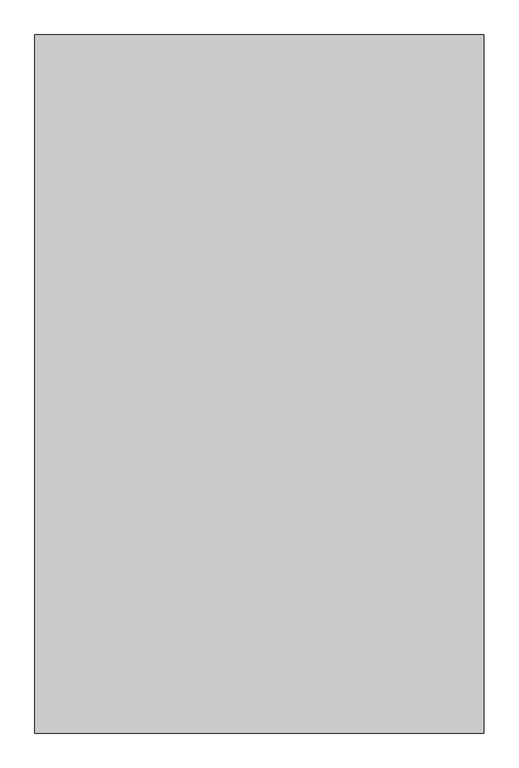
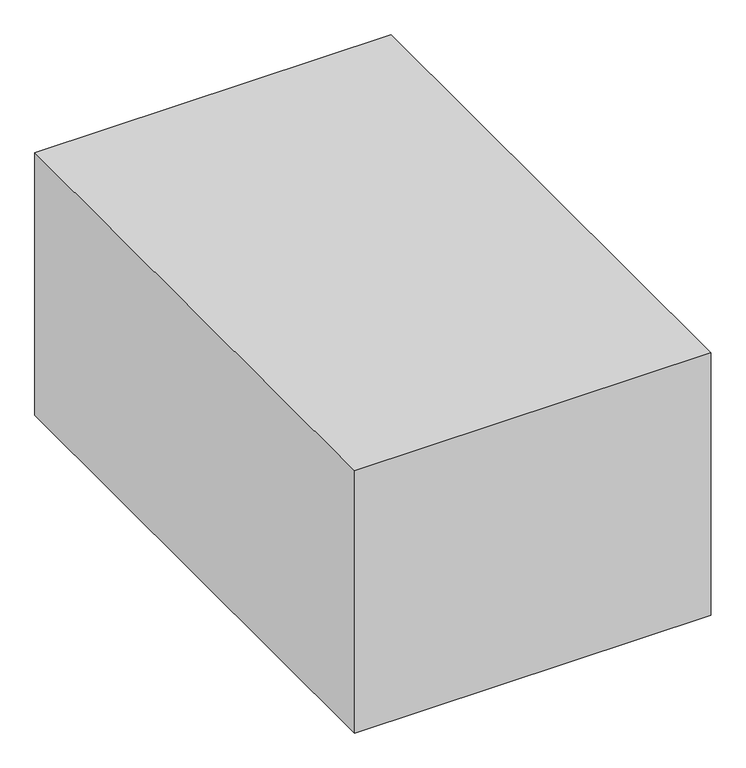
"""IFC4 building model written with IfcOpenShell, lengths in millimetres: proxy geometry, Space Planning Box_hec : Space Planning Box_hec."""

import ifcopenshell
import ifcopenshell.guid

model = None  # the IFC model being written
_history = None  # IfcOwnerHistory: only IFC2X3 demands one
_inside = {}  # id of a spatial element -> (the spatial element, [elements in it])
_under = {}  # id of a project, library or spatial element -> (it, [spatial elements below it])
_declared = {}  # id of a project -> (the project, [libraries it declares])
_typed = {}  # id of a type object -> (the type object, [elements of that type])
_made_of = {}  # id of a material, layer set ... -> (it, [elements and type objects made of it])


def new_model(schema):
    """Start an empty IFC model of exactly this schema.

    Asked for "IFC4X3", IfcOpenShell would pick the latest addendum, in which some entities
    have other attributes; the version numbers below select the first issue.
    IFC2X3 requires an IfcOwnerHistory on every rooted entity: one is made here for all.
    """
    global model, _history
    if schema == "IFC4X3":
        model = ifcopenshell.file(schema_version=(4, 3, 0, 0))
    else:
        model = ifcopenshell.file(schema=schema)
    _inside.clear()
    _under.clear()
    _declared.clear()
    _typed.clear()
    _made_of.clear()
    _history = None
    if model.schema == "IFC2X3":
        org = make("IfcOrganization", Name="unknown")
        user = make(
            "IfcPersonAndOrganization",
            ThePerson=make("IfcPerson", FamilyName="unknown"),
            TheOrganization=org,
        )
        app = make(
            "IfcApplication",
            ApplicationDeveloper=org,
            Version="unknown",
            ApplicationFullName="unknown",
            ApplicationIdentifier="unknown",
        )
        _history = make(
            "IfcOwnerHistory",
            OwningUser=user,
            OwningApplication=app,
            ChangeAction="ADDED",
            CreationDate=0,
        )
    return model


def make(cls, **values):
    """One entity of the class cls with the attributes given. An attribute that is None is left unset."""
    return model.create_entity(
        cls, **{name: value for name, value in values.items() if value is not None}
    )


def rooted(cls, **values):
    """An entity with a GlobalId (a new one), such as an element, a storey or a relation."""
    return make(cls, GlobalId=ifcopenshell.guid.new(), OwnerHistory=_history, **values)


def si_unit(unit_type, name, prefix=None):
    """IfcSIUnit, for example si_unit("LENGTHUNIT", "METRE", prefix="MILLI")."""
    return make("IfcSIUnit", UnitType=unit_type, Prefix=prefix, Name=name)


def assignment(units):
    """IfcUnitAssignment: the units of a project."""
    return None if units is None else make("IfcUnitAssignment", Units=units)


def point(xyz):
    """IfcCartesianPoint."""
    return None if xyz is None else make("IfcCartesianPoint", Coordinates=xyz)


def direction(xyz):
    """IfcDirection."""
    return None if xyz is None else make("IfcDirection", DirectionRatios=xyz)


def frame(location, z_axis=None, x_axis=None):
    """IfcAxis2Placement3D, a coordinate frame: its origin and axes. An axis left out is left unset."""
    return make(
        "IfcAxis2Placement3D",
        Location=point(location),
        Axis=direction(z_axis),
        RefDirection=direction(x_axis),
    )


def origin():
    """The frame at (0, 0, 0) with its axes left unset."""
    return frame((0.0, 0.0, 0.0))


def origin_with_axes():
    """The frame at (0, 0, 0) with the z axis (0, 0, 1) and the x axis (1, 0, 0) written out."""
    return frame((0.0, 0.0, 0.0), z_axis=(0.0, 0.0, 1.0), x_axis=(1.0, 0.0, 0.0))


def place(relative_to, where):
    """IfcLocalPlacement: puts the frame where relative to a parent placement (None: the world)."""
    return make(
        "IfcLocalPlacement", PlacementRelTo=relative_to, RelativePlacement=where
    )


def context(
    kind, dimensions, precision=None, world=None, true_north=None, identifier=None
):
    """IfcGeometricRepresentationContext, for example the 3D "Model" context."""
    return make(
        "IfcGeometricRepresentationContext",
        ContextIdentifier=identifier,
        ContextType=kind,
        CoordinateSpaceDimension=dimensions,
        Precision=precision,
        WorldCoordinateSystem=world,
        TrueNorth=true_north,
    )


def project(units=None, contexts=None):
    """IfcProject with its units and contexts."""
    return rooted(
        "IfcProject",
        Name="project",
        RepresentationContexts=contexts,
        UnitsInContext=assignment(units),
    )


def spatial(cls, under=None, at=None, **own):
    """A site, building, storey or space (cls), placed at a placement, below another one or the project."""
    s = rooted(cls, ObjectPlacement=at, **own)
    if under is not None:
        _under.setdefault(under.id(), (under, []))[1].append(s)
    return s


def polyline(points):
    """IfcPolyline through the points."""
    return make("IfcPolyline", Points=[point(p) for p in points])


def outline(outer, holes=None, kind="AREA"):
    """IfcArbitraryClosedProfileDef: a profile drawn as a closed curve; with holes, ...WithVoids."""
    if holes is None:
        return make("IfcArbitraryClosedProfileDef", ProfileType=kind, OuterCurve=outer)
    return make(
        "IfcArbitraryProfileDefWithVoids",
        ProfileType=kind,
        OuterCurve=outer,
        InnerCurves=holes,
    )


def extrude(swept, where, along, depth):
    """IfcExtrudedAreaSolid: the profile swept, set in the frame where, extruded along a direction by depth."""
    return make(
        "IfcExtrudedAreaSolid",
        SweptArea=swept,
        Position=where,
        ExtrudedDirection=direction(along),
        Depth=depth,
    )


def shape(context_of_items, identifier, shape_type, items):
    """IfcShapeRepresentation: the items that make up one representation, for example the "Body"."""
    return make(
        "IfcShapeRepresentation",
        ContextOfItems=context_of_items,
        RepresentationIdentifier=identifier,
        RepresentationType=shape_type,
        Items=items,
    )


def source(mapping_origin, context_of_items, identifier, shape_type, items):
    """IfcRepresentationMap: a shape defined once, which mapped items show again and again."""
    return make(
        "IfcRepresentationMap",
        MappingOrigin=mapping_origin,
        MappedRepresentation=shape(context_of_items, identifier, shape_type, items),
    )


def transform(
    local_origin,
    x_axis=None,
    y_axis=None,
    z_axis=None,
    scale=None,
    scale2=None,
    scale3=None,
    uniform=True,
):
    """IfcCartesianTransformationOperator3D, or its non-uniform kind. x_axis, y_axis, z_axis: its Axis1, 2, 3."""
    if uniform:
        return make(
            "IfcCartesianTransformationOperator3D",
            Axis1=direction(x_axis),
            Axis2=direction(y_axis),
            LocalOrigin=point(local_origin),
            Scale=scale,
            Axis3=direction(z_axis),
        )
    return make(
        "IfcCartesianTransformationOperator3DnonUniform",
        Axis1=direction(x_axis),
        Axis2=direction(y_axis),
        LocalOrigin=point(local_origin),
        Scale=scale,
        Axis3=direction(z_axis),
        Scale2=scale2,
        Scale3=scale3,
    )


def mapped(mapping_source, mapping_target):
    """IfcMappedItem: shows the shape of a source again, moved by a transform."""
    return make(
        "IfcMappedItem", MappingSource=mapping_source, MappingTarget=mapping_target
    )


def made_of(thing, what):
    """Note that an element or type object is made of a material, layer set ...; save() writes the relation."""
    if what is not None:
        _made_of.setdefault(what.id(), (what, []))[1].append(thing)
    return thing


def element(
    cls,
    number,
    at=None,
    inside=None,
    cuts=None,
    type_object=None,
    material=None,
    context=None,
    identifier="Body",
    shape_type=None,
    held_by="IfcProductDefinitionShape",
    body=None,
    shapes=None,
    **own,
):
    """One element of the class cls, such as IfcWall. Its Tag is "e" and its number.

    at: its placement. inside: the storey or other place that contains it. cuts: it is an
    opening in that element (IfcRelVoidsElement). A single representation is given by context,
    identifier, shape_type and body (its items); several are given by shapes. held_by: the class
    of the entity that holds the representations. save() writes the other relations.
    """
    e = rooted(cls, Tag="e%d" % number, ObjectPlacement=at, **own)
    if body is not None:
        shapes = [shape(context, identifier, shape_type, body)]
    if shapes is not None:
        e.Representation = make(held_by, Representations=shapes)
    if inside is not None:
        _inside.setdefault(inside.id(), (inside, []))[1].append(e)
    if cuts is not None:
        rooted(
            "IfcRelVoidsElement", RelatingBuildingElement=cuts, RelatedOpeningElement=e
        )
    if type_object is not None:
        _typed.setdefault(type_object.id(), (type_object, []))[1].append(e)
    return made_of(e, material)


def aggregate(whole, parts):
    """IfcRelAggregates: a whole, such as a stair, and the parts it consists of."""
    return rooted("IfcRelAggregates", RelatingObject=whole, RelatedObjects=parts)


def save(model, path):
    """Write the relations noted so far, then the file.

    IfcRelAggregates (storeys below a building ...), IfcRelContainedInSpatialStructure (elements
    in a storey), IfcRelDefinesByType, IfcRelAssociatesMaterial and IfcRelDeclares: one each for
    every whole, place, type object, material and project.
    """
    for whole, parts in _under.values():
        aggregate(whole, parts)
    for where, things in _inside.values():
        rooted(
            "IfcRelContainedInSpatialStructure",
            RelatedElements=things,
            RelatingStructure=where,
        )
    for kind, things in _typed.values():
        rooted("IfcRelDefinesByType", RelatedObjects=things, RelatingType=kind)
    for what, things in _made_of.values():
        rooted("IfcRelAssociatesMaterial", RelatedObjects=things, RelatingMaterial=what)
    for by, libraries in _declared.values():
        rooted("IfcRelDeclares", RelatingContext=by, RelatedDefinitions=libraries)
    model.write(path)


def generic_models_10b6925f(model_context):
    return source(origin(), model_context, "Body", "SweptSolid", [
        extrude(outline(polyline([(2250.0, 3500.0), (2250.0, -3500.0), (-2250.0, -3500.0), (-2250.0, 3500.0), (2250.0, 3500.0)])), origin_with_axes(), (0.0, 0.0, 1.0), 3500.0),
    ])


if __name__ == "__main__":
    model = new_model("IFC4")
    model_context = context("Model", 3, world=origin())
    ifc_project = project(units=[si_unit("LENGTHUNIT", "METRE", prefix="MILLI")], contexts=[model_context])
    site = spatial("IfcSite", under=ifc_project)
    building = spatial("IfcBuilding", under=site)
    placement = place(None, origin())
    generic_models_shape = generic_models_10b6925f(model_context)
    element("IfcBuildingElementProxy", 1, Name="Space Planning Box_hec : Space Planning Box_hec", ObjectType="Space Planning Box_hec : Space Planning Box_hec", at=placement, inside=building, context=model_context, shape_type="MappedRepresentation", body=[
        mapped(generic_models_shape, transform((0.0, 0.0, 0.0), x_axis=(1.0, 0.0, 0.0), y_axis=(0.0, 1.0, 0.0), z_axis=(0.0, 0.0, 1.0))),
    ])
    save(model, "model.ifc")

# Revit data of these elements
# Type "Space Planning Box_hec : Space Planning Box_hec"
#   Type Comments = "..."
#   Room Name [instance default] = "?"
#   Interior Finish [instance default] = ""
#   Exterior Finish [instance default] = ""
#   Department [instance default] = ""
#   Assembly Code = "..."
#   Width [instance default] = 1524 mm
#   Program Area [instance default] = 0.00 m²
#   Length [instance default] = 1524 mm
#   Height [instance default] = 1524 mm
#   Area [instance default] = 2.32258 m²
#   Fill Color [instance default] = Cyan
#   Default Elevation = 0
# Element 1 (IfcBuildingElementProxy, "Space Planning Box_hec : Space Planning Box_hec")
#   Room Name = "Break Room"
#   Department = "AR"
#   Width = 4500 mm
#   Program Area = 31.50 m²
#   Length = 7000 mm
#   Height = 3500 mm
#   Area = 31.50 m²
#   Materials on its faces: "Cyan"
# Materials
#   "Cyan": class "Generic", colour RGB 0 255 255, transparency 0.2, Cost = 0
